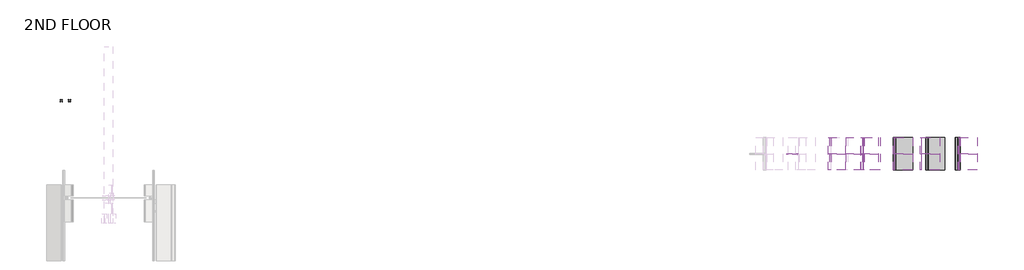
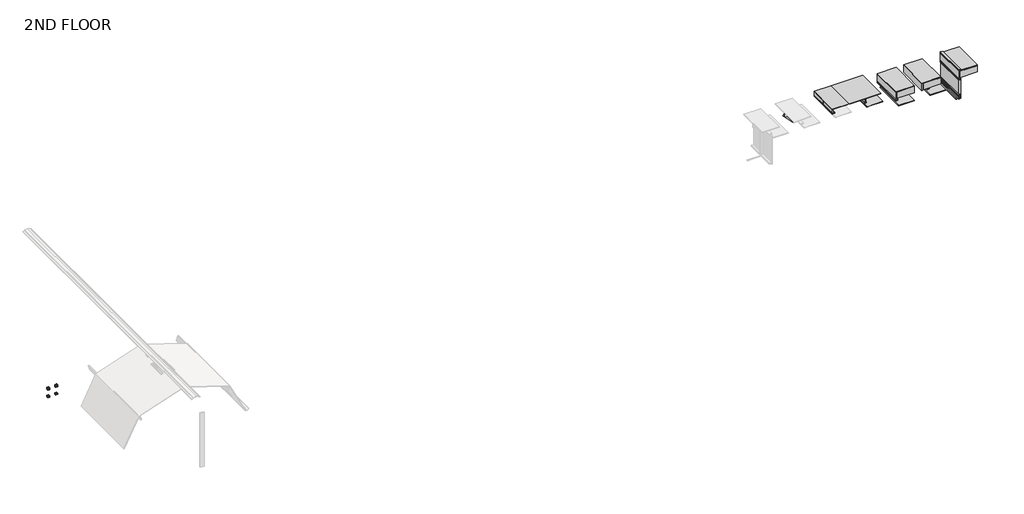
# One storey, part 2 of 2: 61 proxies.
"""IFC4 building model written with IfcOpenShell, lengths in millimetres."""

import ifcopenshell
import ifcopenshell.guid

model = None  # the IFC model being written
_history = None  # IfcOwnerHistory: only IFC2X3 demands one
_inside = {}  # id of a spatial element -> (the spatial element, [elements in it])
_under = {}  # id of a project, library or spatial element -> (it, [spatial elements below it])
_declared = {}  # id of a project -> (the project, [libraries it declares])
_typed = {}  # id of a type object -> (the type object, [elements of that type])
_made_of = {}  # id of a material, layer set ... -> (it, [elements and type objects made of it])


def new_model(schema):
    """Start an empty IFC model of exactly this schema.

    Asked for "IFC4X3", IfcOpenShell would pick the latest addendum, in which some entities
    have other attributes; the version numbers below select the first issue.
    IFC2X3 requires an IfcOwnerHistory on every rooted entity: one is made here for all.
    """
    global model, _history
    if schema == "IFC4X3":
        model = ifcopenshell.file(schema_version=(4, 3, 0, 0))
    else:
        model = ifcopenshell.file(schema=schema)
    _inside.clear()
    _under.clear()
    _declared.clear()
    _typed.clear()
    _made_of.clear()
    _history = None
    if model.schema == "IFC2X3":
        org = make("IfcOrganization", Name="unknown")
        user = make(
            "IfcPersonAndOrganization",
            ThePerson=make("IfcPerson", FamilyName="unknown"),
            TheOrganization=org,
        )
        app = make(
            "IfcApplication",
            ApplicationDeveloper=org,
            Version="unknown",
            ApplicationFullName="unknown",
            ApplicationIdentifier="unknown",
        )
        _history = make(
            "IfcOwnerHistory",
            OwningUser=user,
            OwningApplication=app,
            ChangeAction="ADDED",
            CreationDate=0,
        )
    return model


def make(cls, **values):
    """One entity of the class cls with the attributes given. An attribute that is None is left unset."""
    return model.create_entity(
        cls, **{name: value for name, value in values.items() if value is not None}
    )


def rooted(cls, **values):
    """An entity with a GlobalId (a new one), such as an element, a storey or a relation."""
    return make(cls, GlobalId=ifcopenshell.guid.new(), OwnerHistory=_history, **values)


def si_unit(unit_type, name, prefix=None):
    """IfcSIUnit, for example si_unit("LENGTHUNIT", "METRE", prefix="MILLI")."""
    return make("IfcSIUnit", UnitType=unit_type, Prefix=prefix, Name=name)


def assignment(units):
    """IfcUnitAssignment: the units of a project."""
    return None if units is None else make("IfcUnitAssignment", Units=units)


def point(xyz):
    """IfcCartesianPoint."""
    return None if xyz is None else make("IfcCartesianPoint", Coordinates=xyz)


def direction(xyz):
    """IfcDirection."""
    return None if xyz is None else make("IfcDirection", DirectionRatios=xyz)


def frame(location, z_axis=None, x_axis=None):
    """IfcAxis2Placement3D, a coordinate frame: its origin and axes. An axis left out is left unset."""
    return make(
        "IfcAxis2Placement3D",
        Location=point(location),
        Axis=direction(z_axis),
        RefDirection=direction(x_axis),
    )


def frame_2d(location, x_axis=None):
    """IfcAxis2Placement2D, a coordinate frame in the plane: its origin and x axis."""
    return make(
        "IfcAxis2Placement2D", Location=point(location), RefDirection=direction(x_axis)
    )


def origin():
    """The frame at (0, 0, 0) with its axes left unset."""
    return frame((0.0, 0.0, 0.0))


def origin_with_axes():
    """The frame at (0, 0, 0) with the z axis (0, 0, 1) and the x axis (1, 0, 0) written out."""
    return frame((0.0, 0.0, 0.0), z_axis=(0.0, 0.0, 1.0), x_axis=(1.0, 0.0, 0.0))


def origin_2d():
    """The frame at (0, 0) in the plane with its x axis left unset."""
    return frame_2d((0.0, 0.0))


def place(relative_to, where):
    """IfcLocalPlacement: puts the frame where relative to a parent placement (None: the world)."""
    return make(
        "IfcLocalPlacement", PlacementRelTo=relative_to, RelativePlacement=where
    )


def context(
    kind, dimensions, precision=None, world=None, true_north=None, identifier=None
):
    """IfcGeometricRepresentationContext, for example the 3D "Model" context."""
    return make(
        "IfcGeometricRepresentationContext",
        ContextIdentifier=identifier,
        ContextType=kind,
        CoordinateSpaceDimension=dimensions,
        Precision=precision,
        WorldCoordinateSystem=world,
        TrueNorth=true_north,
    )


def project(units=None, contexts=None):
    """IfcProject with its units and contexts."""
    return rooted(
        "IfcProject",
        Name="project",
        RepresentationContexts=contexts,
        UnitsInContext=assignment(units),
    )


def spatial(cls, under=None, at=None, **own):
    """A site, building, storey or space (cls), placed at a placement, below another one or the project."""
    s = rooted(cls, ObjectPlacement=at, **own)
    if under is not None:
        _under.setdefault(under.id(), (under, []))[1].append(s)
    return s


def polyline(points):
    """IfcPolyline through the points."""
    return make("IfcPolyline", Points=[point(p) for p in points])


def circle_curve(where, radius):
    """IfcCircle in the frame where."""
    return make("IfcCircle", Position=where, Radius=radius)


def trimmed(basis, trim1, trim2, sense, master):
    """IfcTrimmedCurve: the piece of a basis curve between two trims."""
    return make(
        "IfcTrimmedCurve",
        BasisCurve=basis,
        Trim1=trim1,
        Trim2=trim2,
        SenseAgreement=sense,
        MasterRepresentation=master,
    )


def segment(curve, same_sense, transition):
    """IfcCompositeCurveSegment."""
    return make(
        "IfcCompositeCurveSegment",
        Transition=transition,
        SameSense=same_sense,
        ParentCurve=curve,
    )


def composite_curve(segments, self_intersect=None):
    """IfcCompositeCurve: segments joined end to end."""
    return make("IfcCompositeCurve", Segments=segments, SelfIntersect=self_intersect)


def outline(outer, holes=None, kind="AREA"):
    """IfcArbitraryClosedProfileDef: a profile drawn as a closed curve; with holes, ...WithVoids."""
    if holes is None:
        return make("IfcArbitraryClosedProfileDef", ProfileType=kind, OuterCurve=outer)
    return make(
        "IfcArbitraryProfileDefWithVoids",
        ProfileType=kind,
        OuterCurve=outer,
        InnerCurves=holes,
    )


def extrude(swept, where, along, depth):
    """IfcExtrudedAreaSolid: the profile swept, set in the frame where, extruded along a direction by depth."""
    return make(
        "IfcExtrudedAreaSolid",
        SweptArea=swept,
        Position=where,
        ExtrudedDirection=direction(along),
        Depth=depth,
    )


def shape(context_of_items, identifier, shape_type, items):
    """IfcShapeRepresentation: the items that make up one representation, for example the "Body"."""
    return make(
        "IfcShapeRepresentation",
        ContextOfItems=context_of_items,
        RepresentationIdentifier=identifier,
        RepresentationType=shape_type,
        Items=items,
    )


def source(mapping_origin, context_of_items, identifier, shape_type, items):
    """IfcRepresentationMap: a shape defined once, which mapped items show again and again."""
    return make(
        "IfcRepresentationMap",
        MappingOrigin=mapping_origin,
        MappedRepresentation=shape(context_of_items, identifier, shape_type, items),
    )


def transform(
    local_origin,
    x_axis=None,
    y_axis=None,
    z_axis=None,
    scale=None,
    scale2=None,
    scale3=None,
    uniform=True,
):
    """IfcCartesianTransformationOperator3D, or its non-uniform kind. x_axis, y_axis, z_axis: its Axis1, 2, 3."""
    if uniform:
        return make(
            "IfcCartesianTransformationOperator3D",
            Axis1=direction(x_axis),
            Axis2=direction(y_axis),
            LocalOrigin=point(local_origin),
            Scale=scale,
            Axis3=direction(z_axis),
        )
    return make(
        "IfcCartesianTransformationOperator3DnonUniform",
        Axis1=direction(x_axis),
        Axis2=direction(y_axis),
        LocalOrigin=point(local_origin),
        Scale=scale,
        Axis3=direction(z_axis),
        Scale2=scale2,
        Scale3=scale3,
    )


def mapped(mapping_source, mapping_target):
    """IfcMappedItem: shows the shape of a source again, moved by a transform."""
    return make(
        "IfcMappedItem", MappingSource=mapping_source, MappingTarget=mapping_target
    )


def made_of(thing, what):
    """Note that an element or type object is made of a material, layer set ...; save() writes the relation."""
    if what is not None:
        _made_of.setdefault(what.id(), (what, []))[1].append(thing)
    return thing


def element(
    cls,
    number,
    at=None,
    inside=None,
    cuts=None,
    type_object=None,
    material=None,
    context=None,
    identifier="Body",
    shape_type=None,
    held_by="IfcProductDefinitionShape",
    body=None,
    shapes=None,
    **own,
):
    """One element of the class cls, such as IfcWall. Its Tag is "e" and its number.

    at: its placement. inside: the storey or other place that contains it. cuts: it is an
    opening in that element (IfcRelVoidsElement). A single representation is given by context,
    identifier, shape_type and body (its items); several are given by shapes. held_by: the class
    of the entity that holds the representations. save() writes the other relations.
    """
    e = rooted(cls, Tag="e%d" % number, ObjectPlacement=at, **own)
    if body is not None:
        shapes = [shape(context, identifier, shape_type, body)]
    if shapes is not None:
        e.Representation = make(held_by, Representations=shapes)
    if inside is not None:
        _inside.setdefault(inside.id(), (inside, []))[1].append(e)
    if cuts is not None:
        rooted(
            "IfcRelVoidsElement", RelatingBuildingElement=cuts, RelatedOpeningElement=e
        )
    if type_object is not None:
        _typed.setdefault(type_object.id(), (type_object, []))[1].append(e)
    return made_of(e, material)


def aggregate(whole, parts):
    """IfcRelAggregates: a whole, such as a stair, and the parts it consists of."""
    return rooted("IfcRelAggregates", RelatingObject=whole, RelatedObjects=parts)


def save(model, path):
    """Write the relations noted so far, then the file.

    IfcRelAggregates (storeys below a building ...), IfcRelContainedInSpatialStructure (elements
    in a storey), IfcRelDefinesByType, IfcRelAssociatesMaterial and IfcRelDeclares: one each for
    every whole, place, type object, material and project.
    """
    for whole, parts in _under.values():
        aggregate(whole, parts)
    for where, things in _inside.values():
        rooted(
            "IfcRelContainedInSpatialStructure",
            RelatedElements=things,
            RelatingStructure=where,
        )
    for kind, things in _typed.values():
        rooted("IfcRelDefinesByType", RelatedObjects=things, RelatingType=kind)
    for what, things in _made_of.values():
        rooted("IfcRelAssociatesMaterial", RelatedObjects=things, RelatingMaterial=what)
    for by, libraries in _declared.values():
        rooted("IfcRelDeclares", RelatingContext=by, RelatedDefinitions=libraries)
    model.write(path)


def generic_models_10_generic_models_1_ea081297(model_context):
    return source(origin(), model_context, "Body", "SweptSolid", [
        extrude(outline(polyline([(49758.6, 0.0), (49720.5, 0.0), (49720.5, 1219.2), (49758.6, 1219.2), (49758.6, 0.0)])), frame((0.0, 0.0, 5507.83125), z_axis=(0.0, 0.0, 1.0), x_axis=(1.0, 0.0, 0.0)), (0.0, 0.0, 1.0), 139.7),
    ])


def generic_models_102_generic_models_1_8a2dd616(model_context):
    return source(origin(), model_context, "Body", "SweptSolid", [
        extrude(outline(composite_curve([segment(polyline([(4498.578125, 52222.4), (4510.823229, 52207.8068534), (4508.6950617, 52206.021109), (4497.282664, 52219.621875), (4414.3677682, 52219.621875)]), True, "CONTINUOUS"), segment(trimmed(circle_curve(frame_2d((4414.4412941, 52217.6381931)), 1.9850441), [point((4414.3677682, 52219.621875))], [point((4412.45625, 52217.6381931))], True, "CARTESIAN"), True, "CONTINUOUS"), segment(polyline([(4412.45625, 52217.6381931), (4412.45625, 52023.9610661)]), True, "CONTINUOUS"), segment(trimmed(circle_curve(frame_2d((4414.4419899, 52023.9610661)), 1.9857399), [point((4412.45625, 52023.9610661))], [point((4414.3365981, 52021.978125))], True, "CARTESIAN"), True, "CONTINUOUS"), segment(polyline([(4414.3365981, 52021.978125), (4497.282664, 52021.978125), (4508.718285, 52035.6065673), (4510.8464522, 52033.820823), (4498.578125, 52019.2), (4414.440625, 52019.2)]), True, "CONTINUOUS"), segment(trimmed(circle_curve(frame_2d((4414.440625, 52023.9625)), 4.7625), [point((4414.440625, 52019.2))], [point((4409.678125, 52023.9625))], False, "CARTESIAN"), True, "CONTINUOUS"), segment(polyline([(4409.678125, 52023.9625), (4409.678125, 52217.6375)]), True, "CONTINUOUS"), segment(trimmed(circle_curve(frame_2d((4414.440625, 52217.6375)), 4.7625), [point((4409.678125, 52217.6375))], [point((4414.440625, 52222.4))], False, "CARTESIAN"), True, "CONTINUOUS"), segment(polyline([(4414.440625, 52222.4), (4498.578125, 52222.4)]), True, "CONTINUOUS")], self_intersect=False)), frame((0.0, 0.0, 0.0), z_axis=(0.0, 1.0, 0.0), x_axis=(0.0, 0.0, 1.0)), (0.0, 0.0, 1.0), 1219.2),
    ])


def generic_models_103_generic_models_1_250a6a11(model_context):
    return source(origin(), model_context, "Body", "SweptSolid", [
        extrude(outline(polyline([(49784.0, 0.0), (49695.1, 0.0), (49695.1, 1219.2), (49784.0, 1219.2), (49784.0, 0.0)])), frame((0.0, 0.0, 5264.15), z_axis=(0.0, 0.0, 1.0), x_axis=(1.0, 0.0, 0.0)), (0.0, 0.0, 1.0), 38.1),
    ])


def generic_models_104_generic_models_1_af33e5d9(model_context):
    return source(origin(), model_context, "Body", "SweptSolid", [
        extrude(outline(polyline([(52206.021109, 0.0), (52117.121109, 0.0), (52117.121109, 1219.2), (52206.021109, 1219.2), (52206.021109, 0.0)])), frame((0.0, 0.0, 4412.45625), z_axis=(0.0, 0.0, 1.0), x_axis=(1.0, 0.0, 0.0)), (0.0, 0.0, 1.0), 38.1),
    ])


def generic_models_108_generic_models_1_496acf5e(model_context):
    return source(origin(), model_context, "Body", "SweptSolid", [
        extrude(outline(polyline([(52216.05, 1219.2), (52216.05, 0.0), (52139.85, 0.0), (52139.85, 1219.2), (52216.05, 1219.2)])), frame((0.0, 0.0, 4570.4125), z_axis=(0.0, 0.0, 1.0), x_axis=(1.0, 0.0, 0.0)), (0.0, 0.0, 1.0), 565.15),
    ])


def generic_models_109_generic_models_1_8619d77b(model_context):
    return source(origin(), model_context, "Body", "SweptSolid", [
        extrude(outline(polyline([(51003.2, 0.0), (50914.3, 0.0), (50914.3, 1219.2), (51003.2, 1219.2), (51003.2, 0.0)])), frame((0.0, 0.0, 5184.378125), z_axis=(0.0, 0.0, 1.0), x_axis=(1.0, 0.0, 0.0)), (0.0, 0.0, 1.0), 38.1),
    ])


def generic_models_110_generic_models_1_6bdce9b6(model_context):
    return source(origin(), model_context, "Body", "SweptSolid", [
        extrude(outline(polyline([(51642.1451407, 1219.2), (51642.1451407, 0.0), (50914.3, 0.0), (50914.3, 1219.2), (51642.1451407, 1219.2)])), frame((0.0, 0.0, 5508.228125), z_axis=(0.0, 0.0, 1.0), x_axis=(1.0, 0.0, 0.0)), (0.0, 0.0, 1.0), 19.05),
    ])


def generic_models_112_generic_models_65_d168d7b0(model_context):
    return source(origin(), model_context, "Body", "SweptSolid", [
        extrude(outline(polyline([(50952.4, 592.1375), (50952.4, 630.2375), (51642.1451407, 630.2375), (51642.1451407, 592.1375), (50952.4, 592.1375)])), frame((0.0, 0.0, 5222.478125), z_axis=(0.0, 0.0, 1.0), x_axis=(1.0, 0.0, 0.0)), (0.0, 0.0, 1.0), 285.75),
    ])


def generic_models_113_generic_models_1_101608ab(model_context):
    return source(origin(), model_context, "Body", "SweptSolid", [
        extrude(outline(polyline([(52171.6, 0.0), (52133.5, 0.0), (52133.5, 1219.2), (52171.6, 1219.2), (52171.6, 0.0)])), frame((0.0, 0.0, 5222.478125), z_axis=(0.0, 0.0, 1.0), x_axis=(1.0, 0.0, 0.0)), (0.0, 0.0, 1.0), 285.75),
    ])


def generic_models_114_generic_models_1_a6fb1c2c(model_context):
    return source(origin(), model_context, "Body", "SweptSolid", [
        extrude(outline(polyline([(51642.1451407, 1219.2), (51642.1451407, 0.0), (50965.9242022, 0.0), (50965.9242022, 1219.2), (51642.1451407, 1219.2)])), frame((0.0, 0.0, 5237.6235034), z_axis=(0.0, 0.0, 1.0), x_axis=(1.0, 0.0, 0.0)), (0.0, 0.0, 1.0), 254.0),
    ])


def generic_models_12_generic_models_46_b8a9a4e8(model_context):
    return source(origin(), model_context, "Body", "SweptSolid", [
        extrude(outline(polyline([(49757.8505137, 0.0), (49721.1284797, 0.0), (49721.1284797, 1219.2), (49757.8505137, 1219.2), (49757.8505137, 0.0)])), frame((0.0, 0.0, 5505.7509163), z_axis=(0.0, 0.0, 1.0), x_axis=(1.0, 0.0, 0.0)), (0.0, 0.0, 1.0), 1.5875),
    ])


def generic_models_13_generic_models_65_9e643fb9(model_context):
    return source(origin(), model_context, "Body", "SweptSolid", [
        extrude(outline(polyline([(49128.3625, 592.1375), (49128.3625, 630.2375), (50347.5625, 630.2375), (50347.5625, 592.1375), (49128.3625, 592.1375)])), frame((0.0, 0.0, 5507.83125), z_axis=(0.0, 0.0, 1.0), x_axis=(1.0, 0.0, 0.0)), (0.0, 0.0, 1.0), 139.7),
    ])


def generic_models_14_generic_models_1_e8c90d4c(model_context):
    return source(origin(), model_context, "Body", "SweptSolid", [
        extrude(outline(polyline([(2277.1204978, 49799.875), (2239.0204978, 49799.875), (2239.0204978, 49825.275), (2240.6079978, 49825.275), (2240.6079978, 49801.4625), (2277.1204978, 49801.4625), (2277.1204978, 49799.875)])), frame((0.0, 0.0, 0.0), z_axis=(0.0, 1.0, 0.0), x_axis=(0.0, 0.0, 1.0)), (0.0, 0.0, 1.0), 1219.2),
    ])


def generic_models_22_generic_models_1_e5767157(model_context):
    return source(origin(), model_context, "Body", "SweptSolid", [
        extrude(outline(polyline([(2409.6091, 49800.66875), (2409.6091, 49799.875), (2407.0592364, 49799.875), (2405.4618473, 49749.075), (2404.6631527, 49749.075), (2403.0657636, 49799.875), (2400.5159, 49799.875), (2400.5159, 49800.66875), (2409.6091, 49800.66875)])), frame((0.0, 565.15, 0.0), z_axis=(0.0, 1.0, 0.0), x_axis=(0.0, 0.0, 1.0)), (0.0, 0.0, 1.0), 12.7),
    ])


def generic_models_233_generic_models_1_ae5bae41(model_context):
    return source(origin(), model_context, "Body", "SweptSolid", [
        extrude(outline(polyline([(48564.8, 0.0), (48475.9, 0.0), (48475.9, 1219.2), (48564.8, 1219.2), (48564.8, 0.0)])), frame((0.0, 0.0, 5467.35), z_axis=(0.0, 0.0, 1.0), x_axis=(1.0, 0.0, 0.0)), (0.0, 0.0, 1.0), 38.1),
    ])


def generic_models_236_generic_models_1_f8917e71(model_context):
    return source(origin(), model_context, "Body", "SweptSolid", [
        extrude(outline(polyline([(48507.65, 0.0), (48469.55, 0.0), (48469.55, 1219.2), (48507.65, 1219.2), (48507.65, 0.0)])), frame((0.0, 0.0, 5507.83125), z_axis=(0.0, 0.0, 1.0), x_axis=(1.0, 0.0, 0.0)), (0.0, 0.0, 1.0), 139.7),
    ])


def generic_models_237_generic_models_65_1df05f16(model_context):
    return source(origin(), model_context, "Body", "SweptSolid", [
        extrude(outline(polyline([(48469.55, 592.1375), (48469.55, 630.2375), (49128.3625, 630.2375), (49128.3625, 592.1375), (48469.55, 592.1375)])), frame((0.0, 0.0, 5507.83125), z_axis=(0.0, 0.0, 1.0), x_axis=(1.0, 0.0, 0.0)), (0.0, 0.0, 1.0), 139.7),
    ])


def generic_models_240_generic_models_1_611786cf(model_context):
    return source(origin(), model_context, "Body", "SweptSolid", [
        extrude(outline(polyline([(49128.3625, 1219.2), (49128.3625, 0.0), (48469.55, 0.0), (48469.55, 1219.2), (49128.3625, 1219.2)])), frame((0.0, 0.0, 5649.9125), z_axis=(0.0, 0.0, 1.0), x_axis=(1.0, 0.0, 0.0)), (0.0, 0.0, 1.0), 19.05),
    ])


def generic_models_267_generic_models_65_11354230(model_context):
    return source(origin(), model_context, "Body", "SweptSolid", [
        extrude(outline(polyline([(0.0, -38.1), (0.0, 0.0), (514.35, 0.0), (514.35, -38.1), (0.0, -38.1)])), frame((47276.4596037, 592.1375, 5202.484661), z_axis=(0.7071067811865633, 0.0, 0.7071067811865317), x_axis=(-0.7071067811865317, 0.0, 0.7071067811865633)), (0.0, 0.0, 1.0), 88.9),
    ])


def generic_models_29_generic_models_1_59087225(model_context):
    return source(origin(), model_context, "Body", "SweptSolid", [
        extrude(outline(polyline([(50347.5625, 1219.2), (50347.5625, 0.0), (49128.3625, 0.0), (49128.3625, 1219.2), (50347.5625, 1219.2)])), frame((0.0, 0.0, 5647.53125), z_axis=(0.0, 0.0, 1.0), x_axis=(1.0, 0.0, 0.0)), (0.0, 0.0, 1.0), 19.05),
    ])


def generic_models_226_generic_models_1_7dc37832(model_context):
    return source(origin(), model_context, "Body", "SweptSolid", [
        extrude(outline(polyline([(5263.35625, 49733.4159), (5263.35625, 49742.5091), (5264.15, 49742.5091), (5264.15, 49739.9592364), (5314.95, 49738.3618473), (5314.95, 49737.5631527), (5264.15, 49735.9657636), (5264.15, 49733.4159), (5263.35625, 49733.4159)])), frame((0.0, 565.15, 0.0), z_axis=(0.0, 1.0, 0.0), x_axis=(0.0, 0.0, 1.0)), (0.0, 0.0, 1.0), 12.7),
    ])


def generic_models_37_generic_models_1_916dd7c6(model_context):
    return source(origin(), model_context, "Body", "SweptSolid", [
        extrude(outline(polyline([(2409.6091, 49675.25625), (2400.5159, 49675.25625), (2400.5159, 49676.05), (2403.0657636, 49676.05), (2404.6631527, 49726.85), (2405.4618473, 49726.85), (2407.0592364, 49676.05), (2409.6091, 49676.05), (2409.6091, 49675.25625)])), frame((0.0, 565.15, 0.0), z_axis=(0.0, 1.0, 0.0), x_axis=(0.0, 0.0, 1.0)), (0.0, 0.0, 1.0), 12.7),
    ])


def generic_models_202_generic_models_1_0ad20a8b(model_context):
    return source(origin(), model_context, "Body", "SweptSolid", [
        extrude(outline(polyline([(2253.330428, 49813.3451407), (2242.217928, 49813.3451407), (2242.217928, 49826.0451407), (2234.280428, 49828.9341545), (2234.280428, 50422.9451407), (2253.330428, 50422.9451407), (2253.330428, 49813.3451407)])), frame((0.0, 0.0, 0.0), z_axis=(0.0, 1.0, 0.0), x_axis=(0.0, 0.0, 1.0)), (0.0, 0.0, 1.0), 1219.2),
    ])


def generic_models_71_generic_models_1_508a995f(model_context):
    return source(origin(), model_context, "Body", "SweptSolid", [
        extrude(outline(polyline([(50952.4, 0.0), (50914.3, 0.0), (50914.3, 1219.2), (50952.4, 1219.2), (50952.4, 0.0)])), frame((0.0, 0.0, 5222.478125), z_axis=(0.0, 0.0, 1.0), x_axis=(1.0, 0.0, 0.0)), (0.0, 0.0, 1.0), 285.75),
    ])


def generic_models_87_generic_models_1_55a64953(model_context):
    return source(origin(), model_context, "Body", "SweptSolid", [
        extrude(outline(polyline([(51968.4, 0.0), (51930.3, 0.0), (51930.3, 1219.2), (51968.4, 1219.2), (51968.4, 0.0)])), frame((0.0, 0.0, 5222.478125), z_axis=(0.0, 0.0, 1.0), x_axis=(1.0, 0.0, 0.0)), (0.0, 0.0, 1.0), 285.75),
    ])


def proxy_ced08073(model_context):
    return source(origin(), model_context, "Body", "SweptSolid", [
        extrude(outline(polyline([(-9.525, -5.4992613), (-9.525, 5.4992613), (0.0, 10.9985226), (9.525, 5.4992613), (9.525, -5.4992613), (0.0, -10.9985226), (-9.525, -5.4992613)])), frame((0.0, 0.0, -26.8882812), z_axis=(0.0, 0.0, 1.0), x_axis=(1.0, 0.0, 0.0)), (0.0, 0.0, 1.0), 12.7),
        extrude(outline(polyline([(-9.525, 5.4992613), (0.0, 10.9985226), (9.525, 5.4992613), (9.525, -5.4992613), (0.0, -10.9985226), (-9.525, -5.4992613), (-9.525, 5.4992613)])), origin_with_axes(), (0.0, 0.0, 1.0), 12.7),
        extrude(outline(composite_curve([segment(trimmed(circle_curve(origin_2d(), 6.35), [point((-6.35, 0.0))], [point((6.35, 0.0))], False, "CARTESIAN"), True, "CONTINUOUS"), segment(trimmed(circle_curve(origin_2d(), 6.35), [point((6.35, 0.0))], [point((-6.35, 0.0))], False, "CARTESIAN"), True, "CONTINUOUS")], self_intersect=False)), frame((0.0, 0.0, -38.1), z_axis=(0.0, 0.0, 1.0), x_axis=(1.0, 0.0, 0.0)), (0.0, 0.0, 1.0), 38.1),
    ])


def proxy_eacf5a22(model_context):
    return source(origin(), model_context, "Body", "SweptSolid", [
        extrude(outline(polyline([(-9.525, 5.4992613), (0.0, 10.9985226), (9.525, 5.4992613), (9.525, -5.4992613), (0.0, -10.9985226), (-9.525, -5.4992613), (-9.525, 5.4992613)])), frame((0.0, 0.0, -61.0195313), z_axis=(0.0, 0.0, 1.0), x_axis=(1.0, 0.0, 0.0)), (0.0, 0.0, 1.0), 8.73125),
        extrude(outline(polyline([(-9.525, -5.4992613), (-9.525, 5.4992613), (0.0, 10.9985226), (9.525, 5.4992613), (9.525, -5.4992613), (0.0, -10.9985226), (-9.525, -5.4992613)])), origin_with_axes(), (0.0, 0.0, 1.0), 8.73125),
        extrude(outline(composite_curve([segment(trimmed(circle_curve(origin_2d(), 6.35), [point((-6.35, 0.0))], [point((6.35, 0.0))], False, "CARTESIAN"), True, "CONTINUOUS"), segment(trimmed(circle_curve(origin_2d(), 6.35), [point((6.35, 0.0))], [point((-6.35, 0.0))], False, "CARTESIAN"), True, "CONTINUOUS")], self_intersect=False)), frame((0.0, 0.0, -63.5), z_axis=(0.0, 0.0, 1.0), x_axis=(1.0, 0.0, 0.0)), (0.0, 0.0, 1.0), 63.5),
    ])


model = new_model("IFC4")

# Units and contexts
model_context = context("Model", 3, world=origin())
ifc_project = project(units=[si_unit("LENGTHUNIT", "METRE", prefix="MILLI")], contexts=[model_context])

# Site, building, storey
site = spatial("IfcSite", under=ifc_project)
building = spatial("IfcBuilding", under=site)
storey = spatial("IfcBuildingStorey", under=building, Name="2ND FLOOR", Elevation=3984.625)

# Proxies
placement = place(None, origin())
generic_models_10_generic_models_1_shape = generic_models_10_generic_models_1_ea081297(model_context)
element("IfcBuildingElementProxy", 1, Name="Generic Models 10 : Generic Models 1", ObjectType="Generic Models 10 : Generic Models 1", at=placement, inside=storey, context=model_context, shape_type="MappedRepresentation", body=[
    mapped(generic_models_10_generic_models_1_shape, transform((0.0, 0.0, 0.0), x_axis=(1.0, 0.0, 0.0), y_axis=(0.0, 1.0, 0.0), z_axis=(0.0, 0.0, 1.0))),
])
generic_models_102_generic_models_1_shape = generic_models_102_generic_models_1_8a2dd616(model_context)
element("IfcBuildingElementProxy", 2, Name="Generic Models 102 : Generic Models 1", ObjectType="Generic Models 102 : Generic Models 1", at=placement, inside=storey, context=model_context, shape_type="MappedRepresentation", body=[
    mapped(generic_models_102_generic_models_1_shape, transform((1219.2, 0.0, 0.0), x_axis=(1.0, 0.0, 0.0), y_axis=(0.0, 1.0, 0.0), z_axis=(0.0, 0.0, 1.0))),
])
generic_models_103_generic_models_1_shape = generic_models_103_generic_models_1_250a6a11(model_context)
element("IfcBuildingElementProxy", 3, Name="Generic Models 103 : Generic Models 1", ObjectType="Generic Models 103 : Generic Models 1", at=placement, inside=storey, context=model_context, shape_type="MappedRepresentation", body=[
    mapped(generic_models_103_generic_models_1_shape, transform((3657.6, 0.0, -892.571875), x_axis=(1.0, 0.0, 0.0), y_axis=(0.0, 1.0, 0.0), z_axis=(0.0, 0.0, 1.0))),
])
generic_models_104_generic_models_1_shape = generic_models_104_generic_models_1_af33e5d9(model_context)
element("IfcBuildingElementProxy", 4, Name="Generic Models 104 : Generic Models 1", ObjectType="Generic Models 104 : Generic Models 1", at=placement, inside=storey, context=model_context, shape_type="MappedRepresentation", body=[
    mapped(generic_models_104_generic_models_1_shape, transform((1219.2, 0.0, 0.0), x_axis=(1.0, 0.0, 0.0), y_axis=(0.0, 1.0, 0.0), z_axis=(0.0, 0.0, 1.0))),
])
element("IfcBuildingElementProxy", 5, Name="Generic Models 105 : Generic Models 1", ObjectType="Generic Models 105 : Generic Models 1", at=placement, inside=storey, context=model_context, shape_type="MappedRepresentation", body=[
    mapped(generic_models_103_generic_models_1_shape, transform((3641.221109, 0.0, -813.59375), x_axis=(1.0, 0.0, 0.0), y_axis=(0.0, 1.0, 0.0), z_axis=(0.0, 0.0, 1.0))),
])
element("IfcBuildingElementProxy", 6, Name="Generic Models 106 : Generic Models 1", ObjectType="Generic Models 106 : Generic Models 1", at=placement, inside=storey, context=model_context, shape_type="MappedRepresentation", body=[
    mapped(generic_models_103_generic_models_1_shape, transform((3641.221109, 0.0, -775.49375), x_axis=(1.0, 0.0, 0.0), y_axis=(0.0, 1.0, 0.0), z_axis=(0.0, 0.0, 1.0))),
])
element("IfcBuildingElementProxy", 7, Name="Generic Models 107 : Generic Models 1", ObjectType="Generic Models 107 : Generic Models 1", at=placement, inside=storey, context=model_context, shape_type="MappedRepresentation", body=[
    mapped(generic_models_103_generic_models_1_shape, transform((3657.6, 0.0, -737.39375), x_axis=(1.0, 0.0, 0.0), y_axis=(0.0, 1.0, 0.0), z_axis=(0.0, 0.0, 1.0))),
])
generic_models_108_generic_models_1_shape = generic_models_108_generic_models_1_496acf5e(model_context)
element("IfcBuildingElementProxy", 8, Name="Generic Models 108 : Generic Models 1", ObjectType="Generic Models 108 : Generic Models 1", at=placement, inside=storey, context=model_context, shape_type="MappedRepresentation", body=[
    mapped(generic_models_108_generic_models_1_shape, transform((1219.2, 0.0, 0.0), x_axis=(1.0, 0.0, 0.0), y_axis=(0.0, 1.0, 0.0), z_axis=(0.0, 0.0, 1.0))),
])
generic_models_109_generic_models_1_shape = generic_models_109_generic_models_1_8619d77b(model_context)
element("IfcBuildingElementProxy", 9, Name="Generic Models 109 : Generic Models 1", ObjectType="Generic Models 109 : Generic Models 1", at=placement, inside=storey, context=model_context, shape_type="MappedRepresentation", body=[
    mapped(generic_models_109_generic_models_1_shape, transform((2438.4, 0.0, 0.0), x_axis=(1.0, 0.0, 0.0), y_axis=(0.0, 1.0, 0.0), z_axis=(0.0, 0.0, 1.0))),
])
generic_models_110_generic_models_1_shape = generic_models_110_generic_models_1_6bdce9b6(model_context)
element("IfcBuildingElementProxy", 10, Name="Generic Models 110 : Generic Models 1", ObjectType="Generic Models 110 : Generic Models 1", at=placement, inside=storey, context=model_context, shape_type="MappedRepresentation", body=[
    mapped(generic_models_110_generic_models_1_shape, transform((2438.4, 0.0, 0.0), x_axis=(1.0, 0.0, 0.0), y_axis=(0.0, 1.0, 0.0), z_axis=(0.0, 0.0, 1.0))),
])
element("IfcBuildingElementProxy", 11, Name="Generic Models 111 : Generic Models 1", ObjectType="Generic Models 111 : Generic Models 1", at=placement, inside=storey, context=model_context, shape_type="MappedRepresentation", body=[
    mapped(generic_models_109_generic_models_1_shape, transform((2438.4, 0.0, -38.1), x_axis=(1.0, 0.0, 0.0), y_axis=(0.0, 1.0, 0.0), z_axis=(0.0, 0.0, 1.0))),
])
generic_models_112_generic_models_65_shape = generic_models_112_generic_models_65_d168d7b0(model_context)
element("IfcBuildingElementProxy", 12, Name="Generic Models 112 : Generic Models 65", ObjectType="Generic Models 112 : Generic Models 65", at=placement, inside=storey, context=model_context, shape_type="MappedRepresentation", body=[
    mapped(generic_models_112_generic_models_65_shape, transform((2438.4, 0.0, 0.0), x_axis=(1.0, 0.0, 0.0), y_axis=(0.0, 1.0, 0.0), z_axis=(0.0, 0.0, 1.0))),
])
generic_models_113_generic_models_1_shape = generic_models_113_generic_models_1_101608ab(model_context)
element("IfcBuildingElementProxy", 13, Name="Generic Models 113 : Generic Models 1", ObjectType="Generic Models 113 : Generic Models 1", at=placement, inside=storey, context=model_context, shape_type="MappedRepresentation", body=[
    mapped(generic_models_113_generic_models_1_shape, transform((1219.2, 0.0, 0.0), x_axis=(1.0, 0.0, 0.0), y_axis=(0.0, 1.0, 0.0), z_axis=(0.0, 0.0, 1.0))),
])
generic_models_114_generic_models_1_shape = generic_models_114_generic_models_1_a6fb1c2c(model_context)
element("IfcBuildingElementProxy", 14, Name="Generic Models 114 : Generic Models 1", ObjectType="Generic Models 114 : Generic Models 1", at=placement, inside=storey, context=model_context, shape_type="MappedRepresentation", body=[
    mapped(generic_models_114_generic_models_1_shape, transform((2438.4, 0.0, 0.0), x_axis=(1.0, 0.0, 0.0), y_axis=(0.0, 1.0, 0.0), z_axis=(0.0, 0.0, 1.0))),
])
element("IfcBuildingElementProxy", 15, Name="Generic Models 115 : Generic Models 1", ObjectType="Generic Models 115 : Generic Models 1", at=placement, inside=storey, context=model_context, shape_type="MappedRepresentation", body=[
    mapped(generic_models_109_generic_models_1_shape, transform((2438.4, 0.0, 342.9), x_axis=(1.0, 0.0, 0.0), y_axis=(0.0, 1.0, 0.0), z_axis=(0.0, 0.0, 1.0))),
])
generic_models_12_generic_models_46_shape = generic_models_12_generic_models_46_b8a9a4e8(model_context)
element("IfcBuildingElementProxy", 16, Name="Generic Models 12 : Generic Models 46", ObjectType="Generic Models 12 : Generic Models 46", at=placement, inside=storey, context=model_context, shape_type="MappedRepresentation", body=[
    mapped(generic_models_12_generic_models_46_shape, transform((0.0, 0.0, 0.0), x_axis=(1.0, 0.0, 0.0), y_axis=(0.0, 1.0, 0.0), z_axis=(0.0, 0.0, 1.0))),
])
generic_models_13_generic_models_65_shape = generic_models_13_generic_models_65_9e643fb9(model_context)
element("IfcBuildingElementProxy", 17, Name="Generic Models 13 : Generic Models 65", ObjectType="Generic Models 13 : Generic Models 65", at=placement, inside=storey, context=model_context, shape_type="MappedRepresentation", body=[
    mapped(generic_models_13_generic_models_65_shape, transform((0.0, 0.0, 0.0), x_axis=(1.0, 0.0, 0.0), y_axis=(0.0, 1.0, 0.0), z_axis=(0.0, 0.0, 1.0))),
])
generic_models_14_generic_models_1_shape = generic_models_14_generic_models_1_e8c90d4c(model_context)
element("IfcBuildingElementProxy", 18, Name="Generic Models 14 : Generic Models 1", ObjectType="Generic Models 14 : Generic Models 1", at=placement, inside=storey, context=model_context, shape_type="MappedRepresentation", body=[
    mapped(generic_models_14_generic_models_1_shape, transform((0.0, 0.0, 3050.778125), x_axis=(1.0, 0.0, 0.0), y_axis=(0.0, 1.0, 0.0), z_axis=(0.0, 0.0, 1.0))),
])
generic_models_22_generic_models_1_shape = generic_models_22_generic_models_1_e5767157(model_context)
element("IfcBuildingElementProxy", 19, Name="Generic Models 22 : Generic Models 1", ObjectType="Generic Models 22 : Generic Models 1", at=placement, inside=storey, context=model_context, shape_type="MappedRepresentation", body=[
    mapped(generic_models_22_generic_models_1_shape, transform((0.0, 0.0, 3081.3375), x_axis=(1.0, 0.0, 0.0), y_axis=(0.0, 1.0, 0.0), z_axis=(0.0, 0.0, 1.0))),
])
generic_models_233_generic_models_1_shape = generic_models_233_generic_models_1_ae5bae41(model_context)
element("IfcBuildingElementProxy", 20, Name="Generic Models 233 : Generic Models 1", ObjectType="Generic Models 233 : Generic Models 1", at=placement, inside=storey, context=model_context, shape_type="MappedRepresentation", body=[
    mapped(generic_models_233_generic_models_1_shape, transform((0.0, 0.0, 0.0), x_axis=(1.0, 0.0, 0.0), y_axis=(0.0, 1.0, 0.0), z_axis=(0.0, 0.0, 1.0))),
])
generic_models_236_generic_models_1_shape = generic_models_236_generic_models_1_f8917e71(model_context)
element("IfcBuildingElementProxy", 21, Name="Generic Models 236 : Generic Models 1", ObjectType="Generic Models 236 : Generic Models 1", at=placement, inside=storey, context=model_context, shape_type="MappedRepresentation", body=[
    mapped(generic_models_236_generic_models_1_shape, transform((0.0, 0.0, 0.0), x_axis=(1.0, 0.0, 0.0), y_axis=(0.0, 1.0, 0.0), z_axis=(0.0, 0.0, 1.0))),
])
generic_models_237_generic_models_65_shape = generic_models_237_generic_models_65_1df05f16(model_context)
element("IfcBuildingElementProxy", 22, Name="Generic Models 237 : Generic Models 65", ObjectType="Generic Models 237 : Generic Models 65", at=placement, inside=storey, context=model_context, shape_type="MappedRepresentation", body=[
    mapped(generic_models_237_generic_models_65_shape, transform((0.0, 0.0, 0.0), x_axis=(1.0, 0.0, 0.0), y_axis=(0.0, 1.0, 0.0), z_axis=(0.0, 0.0, 1.0))),
])
generic_models_240_generic_models_1_shape = generic_models_240_generic_models_1_611786cf(model_context)
element("IfcBuildingElementProxy", 23, Name="Generic Models 240 : Generic Models 1", ObjectType="Generic Models 240 : Generic Models 1", at=placement, inside=storey, context=model_context, shape_type="MappedRepresentation", body=[
    mapped(generic_models_240_generic_models_1_shape, transform((0.0, 0.0, 0.0), x_axis=(1.0, 0.0, 0.0), y_axis=(0.0, 1.0, 0.0), z_axis=(0.0, 0.0, 1.0))),
])
element("IfcBuildingElementProxy", 24, Name="Generic Models 25 : Generic Models 46", ObjectType="Generic Models 25 : Generic Models 46", at=placement, inside=storey, context=model_context, shape_type="MappedRepresentation", body=[
    mapped(generic_models_12_generic_models_46_shape, transform((0.0, 0.0, 142.08125), x_axis=(1.0, 0.0, 0.0), y_axis=(0.0, 1.0, 0.0), z_axis=(0.0, 0.0, 1.0))),
])
generic_models_267_generic_models_65_shape = generic_models_267_generic_models_65_11354230(model_context)
element("IfcBuildingElementProxy", 25, Name="Generic Models 267 : Generic Models 65", ObjectType="Generic Models 267 : Generic Models 65", at=placement, inside=storey, context=model_context, shape_type="MappedRepresentation", body=[
    mapped(generic_models_267_generic_models_65_shape, transform((0.0, 0.0, 0.0), x_axis=(1.0, 0.0, 0.0), y_axis=(0.0, 1.0, 0.0), z_axis=(0.0, 0.0, 1.0))),
])
generic_models_29_generic_models_1_shape = generic_models_29_generic_models_1_59087225(model_context)
element("IfcBuildingElementProxy", 26, Name="Generic Models 29 : Generic Models 1", ObjectType="Generic Models 29 : Generic Models 1", at=placement, inside=storey, context=model_context, shape_type="MappedRepresentation", body=[
    mapped(generic_models_29_generic_models_1_shape, transform((0.0, 0.0, 2.38125), x_axis=(1.0, 0.0, 0.0), y_axis=(0.0, 1.0, 0.0), z_axis=(0.0, 0.0, 1.0))),
])
generic_models_226_generic_models_1_shape = generic_models_226_generic_models_1_7dc37832(model_context)
element("IfcBuildingElementProxy", 27, Name="Generic Models 39 : Generic Models 1", ObjectType="Generic Models 39 : Generic Models 1", at=placement, inside=storey, context=model_context, shape_type="MappedRepresentation", body=[
    mapped(generic_models_226_generic_models_1_shape, transform((0.0, 0.0, 203.2), x_axis=(1.0, 0.0, 0.0), y_axis=(0.0, 1.0, 0.0), z_axis=(0.0, 0.0, 1.0))),
])
generic_models_37_generic_models_1_shape = generic_models_37_generic_models_1_916dd7c6(model_context)
element("IfcBuildingElementProxy", 28, Name="Generic Models 47 : Generic Models 1", ObjectType="Generic Models 47 : Generic Models 1", at=placement, inside=storey, context=model_context, shape_type="MappedRepresentation", body=[
    mapped(generic_models_37_generic_models_1_shape, transform((3.175, 0.0, 3081.3375), x_axis=(1.0, 0.0, 0.0), y_axis=(0.0, 1.0, 0.0), z_axis=(0.0, 0.0, 1.0))),
])
generic_models_202_generic_models_1_shape = generic_models_202_generic_models_1_0ad20a8b(model_context)
element("IfcBuildingElementProxy", 29, Name="Generic Models 49 : Generic Models 1", ObjectType="Generic Models 49 : Generic Models 1", at=placement, inside=storey, context=model_context, shape_type="MappedRepresentation", body=[
    mapped(generic_models_202_generic_models_1_shape, transform((0.0, 0.0, 3050.778125), x_axis=(1.0, 0.0, 0.0), y_axis=(0.0, 1.0, 0.0), z_axis=(0.0, 0.0, 1.0))),
])
element("IfcBuildingElementProxy", 30, Name="Generic Models 54 : Generic Models 1", ObjectType="Generic Models 54 : Generic Models 1", at=placement, inside=storey, context=model_context, shape_type="MappedRepresentation", body=[
    mapped(generic_models_14_generic_models_1_shape, transform((1219.2, 0.0, 2676.128125), x_axis=(1.0, 0.0, 0.0), y_axis=(0.0, 1.0, 0.0), z_axis=(0.0, 0.0, 1.0))),
])
element("IfcBuildingElementProxy", 31, Name="Generic Models 59 : Generic Models 65", ObjectType="Generic Models 59 : Generic Models 65", at=placement, inside=storey, context=model_context, shape_type="MappedRepresentation", body=[
    mapped(generic_models_112_generic_models_65_shape, transform((0.0, 0.0, 0.0), x_axis=(1.0, 0.0, 0.0), y_axis=(0.0, 1.0, 0.0), z_axis=(0.0, 0.0, 1.0))),
])
element("IfcBuildingElementProxy", 32, Name="Generic Models 6 : Generic Models 1", ObjectType="Generic Models 6 : Generic Models 1", at=placement, inside=storey, context=model_context, shape_type="MappedRepresentation", body=[
    mapped(generic_models_103_generic_models_1_shape, transform((0.0, 0.0, 203.2), x_axis=(1.0, 0.0, 0.0), y_axis=(0.0, 1.0, 0.0), z_axis=(0.0, 0.0, 1.0))),
])
element("IfcBuildingElementProxy", 33, Name="Generic Models 62 : Generic Models 1", ObjectType="Generic Models 62 : Generic Models 1", at=placement, inside=storey, context=model_context, shape_type="MappedRepresentation", body=[
    mapped(generic_models_202_generic_models_1_shape, transform((1219.2, 0.0, 2676.128125), x_axis=(1.0, 0.0, 0.0), y_axis=(0.0, 1.0, 0.0), z_axis=(0.0, 0.0, 1.0))),
])
element("IfcBuildingElementProxy", 34, Name="Generic Models 64 : Generic Models 1", ObjectType="Generic Models 64 : Generic Models 1", at=placement, inside=storey, context=model_context, shape_type="MappedRepresentation", body=[
    mapped(generic_models_109_generic_models_1_shape, transform((0.0, 0.0, 0.0), x_axis=(1.0, 0.0, 0.0), y_axis=(0.0, 1.0, 0.0), z_axis=(0.0, 0.0, 1.0))),
])
element("IfcBuildingElementProxy", 35, Name="Generic Models 66 : Generic Models 1", ObjectType="Generic Models 66 : Generic Models 1", at=placement, inside=storey, context=model_context, shape_type="MappedRepresentation", body=[
    mapped(generic_models_110_generic_models_1_shape, transform((0.0, 0.0, 0.0), x_axis=(1.0, 0.0, 0.0), y_axis=(0.0, 1.0, 0.0), z_axis=(0.0, 0.0, 1.0))),
])
element("IfcBuildingElementProxy", 36, Name="Generic Models 70 : Generic Models 1", ObjectType="Generic Models 70 : Generic Models 1", at=placement, inside=storey, context=model_context, shape_type="MappedRepresentation", body=[
    mapped(generic_models_109_generic_models_1_shape, transform((0.0, 0.0, -38.1), x_axis=(1.0, 0.0, 0.0), y_axis=(0.0, 1.0, 0.0), z_axis=(0.0, 0.0, 1.0))),
])
generic_models_71_generic_models_1_shape = generic_models_71_generic_models_1_508a995f(model_context)
element("IfcBuildingElementProxy", 37, Name="Generic Models 71 : Generic Models 1", ObjectType="Generic Models 71 : Generic Models 1", at=placement, inside=storey, context=model_context, shape_type="MappedRepresentation", body=[
    mapped(generic_models_71_generic_models_1_shape, transform((0.0, 0.0, 0.0), x_axis=(1.0, 0.0, 0.0), y_axis=(0.0, 1.0, 0.0), z_axis=(0.0, 0.0, 1.0))),
])
element("IfcBuildingElementProxy", 38, Name="Generic Models 72 : Generic Models 1", ObjectType="Generic Models 72 : Generic Models 1", at=placement, inside=storey, context=model_context, shape_type="MappedRepresentation", body=[
    mapped(generic_models_114_generic_models_1_shape, transform((0.0, 0.0, 0.0), x_axis=(1.0, 0.0, 0.0), y_axis=(0.0, 1.0, 0.0), z_axis=(0.0, 0.0, 1.0))),
])
element("IfcBuildingElementProxy", 39, Name="Generic Models 75 : Generic Models 1", ObjectType="Generic Models 75 : Generic Models 1", at=placement, inside=storey, context=model_context, shape_type="MappedRepresentation", body=[
    mapped(generic_models_14_generic_models_1_shape, transform((2438.4, 0.0, 2676.128125), x_axis=(1.0, 0.0, 0.0), y_axis=(0.0, 1.0, 0.0), z_axis=(0.0, 0.0, 1.0))),
])
element("IfcBuildingElementProxy", 40, Name="Generic Models 79 : Generic Models 1", ObjectType="Generic Models 79 : Generic Models 1", at=placement, inside=storey, context=model_context, shape_type="MappedRepresentation", body=[
    mapped(generic_models_202_generic_models_1_shape, transform((2438.4, 0.0, 2676.128125), x_axis=(1.0, 0.0, 0.0), y_axis=(0.0, 1.0, 0.0), z_axis=(0.0, 0.0, 1.0))),
])
element("IfcBuildingElementProxy", 41, Name="Generic Models 81 : Generic Models 1", ObjectType="Generic Models 81 : Generic Models 1", at=placement, inside=storey, context=model_context, shape_type="MappedRepresentation", body=[
    mapped(generic_models_109_generic_models_1_shape, transform((1219.2, 0.0, 0.0), x_axis=(1.0, 0.0, 0.0), y_axis=(0.0, 1.0, 0.0), z_axis=(0.0, 0.0, 1.0))),
])
element("IfcBuildingElementProxy", 42, Name="Generic Models 82 : Generic Models 1", ObjectType="Generic Models 82 : Generic Models 1", at=placement, inside=storey, context=model_context, shape_type="MappedRepresentation", body=[
    mapped(generic_models_110_generic_models_1_shape, transform((1016.0, 0.0, 0.0), x_axis=(1.0, 0.0, 0.0), y_axis=(0.0, 1.0, 0.0), z_axis=(0.0, 0.0, 1.0))),
])
element("IfcBuildingElementProxy", 43, Name="Generic Models 86 : Generic Models 65", ObjectType="Generic Models 86 : Generic Models 65", at=placement, inside=storey, context=model_context, shape_type="MappedRepresentation", body=[
    mapped(generic_models_112_generic_models_65_shape, transform((1016.0, 0.0, 0.0), x_axis=(1.0, 0.0, 0.0), y_axis=(0.0, 1.0, 0.0), z_axis=(0.0, 0.0, 1.0))),
])
generic_models_87_generic_models_1_shape = generic_models_87_generic_models_1_55a64953(model_context)
element("IfcBuildingElementProxy", 44, Name="Generic Models 87 : Generic Models 1", ObjectType="Generic Models 87 : Generic Models 1", at=placement, inside=storey, context=model_context, shape_type="MappedRepresentation", body=[
    mapped(generic_models_87_generic_models_1_shape, transform((0.0, 0.0, 0.0), x_axis=(1.0, 0.0, 0.0), y_axis=(0.0, 1.0, 0.0), z_axis=(0.0, 0.0, 1.0))),
])
element("IfcBuildingElementProxy", 45, Name="Generic Models 88 : Generic Models 1", ObjectType="Generic Models 88 : Generic Models 1", at=placement, inside=storey, context=model_context, shape_type="MappedRepresentation", body=[
    mapped(generic_models_114_generic_models_1_shape, transform((1016.0, 0.0, 0.0), x_axis=(1.0, 0.0, 0.0), y_axis=(0.0, 1.0, 0.0), z_axis=(0.0, 0.0, 1.0))),
])
proxy_shape = proxy_ced08073(model_context)
element("IfcBuildingElementProxy", 46, Name="Lag Bolt : 1/2\" X 1 1/2\"", ObjectType="Lag Bolt : 1/2\" X 1 1/2\"", at=placement, inside=storey, context=model_context, shape_type="MappedRepresentation", body=[
    mapped(proxy_shape, transform((19698.4870052, 2642.8615366, 2431.4546875), x_axis=(1.0, 0.0, 0.0), y_axis=(0.0, -1.0, 0.0), z_axis=(0.0, 0.0, -1.0))),
])
element("IfcBuildingElementProxy", 47, Name="Lag Bolt : 1/2\" X 1 1/2\"", ObjectType="Lag Bolt : 1/2\" X 1 1/2\"", at=placement, inside=storey, context=model_context, shape_type="MappedRepresentation", body=[
    mapped(proxy_shape, transform((19634.9870052, 2642.8615366, 2431.4546875), x_axis=(1.0, 0.0, 0.0), y_axis=(0.0, -1.0, 0.0), z_axis=(0.0, 0.0, -1.0))),
])
element("IfcBuildingElementProxy", 48, Name="Lag Bolt : 1/2\" X 1 1/2\"", ObjectType="Lag Bolt : 1/2\" X 1 1/2\"", at=placement, inside=storey, context=model_context, shape_type="MappedRepresentation", body=[
    mapped(proxy_shape, transform((19698.4870052, 2579.3615366, 2431.4546875), x_axis=(1.0, 0.0, 0.0), y_axis=(0.0, -1.0, 0.0), z_axis=(0.0, 0.0, -1.0))),
])
element("IfcBuildingElementProxy", 49, Name="Lag Bolt : 1/2\" X 1 1/2\"", ObjectType="Lag Bolt : 1/2\" X 1 1/2\"", at=placement, inside=storey, context=model_context, shape_type="MappedRepresentation", body=[
    mapped(proxy_shape, transform((19634.9870052, 2579.3615366, 2431.4546875), x_axis=(1.0, 0.0, 0.0), y_axis=(0.0, -1.0, 0.0), z_axis=(0.0, 0.0, -1.0))),
])
element("IfcBuildingElementProxy", 50, Name="Lag Bolt : 1/2\" X 1 1/2\"", ObjectType="Lag Bolt : 1/2\" X 1 1/2\"", at=placement, inside=storey, context=model_context, shape_type="MappedRepresentation", body=[
    mapped(proxy_shape, transform((20003.2870052, 2642.8615366, 2431.4546875), x_axis=(1.0, 0.0, 0.0), y_axis=(0.0, -1.0, 0.0), z_axis=(0.0, 0.0, -1.0))),
])
element("IfcBuildingElementProxy", 51, Name="Lag Bolt : 1/2\" X 1 1/2\"", ObjectType="Lag Bolt : 1/2\" X 1 1/2\"", at=placement, inside=storey, context=model_context, shape_type="MappedRepresentation", body=[
    mapped(proxy_shape, transform((19939.7870052, 2642.8615366, 2431.4546875), x_axis=(1.0, 0.0, 0.0), y_axis=(0.0, -1.0, 0.0), z_axis=(0.0, 0.0, -1.0))),
])
element("IfcBuildingElementProxy", 52, Name="Lag Bolt : 1/2\" X 1 1/2\"", ObjectType="Lag Bolt : 1/2\" X 1 1/2\"", at=placement, inside=storey, context=model_context, shape_type="MappedRepresentation", body=[
    mapped(proxy_shape, transform((20003.2870052, 2579.3615366, 2431.4546875), x_axis=(1.0, 0.0, 0.0), y_axis=(0.0, -1.0, 0.0), z_axis=(0.0, 0.0, -1.0))),
])
element("IfcBuildingElementProxy", 53, Name="Lag Bolt : 1/2\" X 1 1/2\"", ObjectType="Lag Bolt : 1/2\" X 1 1/2\"", at=placement, inside=storey, context=model_context, shape_type="MappedRepresentation", body=[
    mapped(proxy_shape, transform((19939.7870052, 2579.3615366, 2431.4546875), x_axis=(1.0, 0.0, 0.0), y_axis=(0.0, -1.0, 0.0), z_axis=(0.0, 0.0, -1.0))),
])
proxy_2_shape = proxy_eacf5a22(model_context)
element("IfcBuildingElementProxy", 54, Name="Lag Bolt : 1/2\" x 2 1/2\"", ObjectType="Lag Bolt : 1/2\" x 2 1/2\"", at=placement, inside=storey, context=model_context, shape_type="MappedRepresentation", body=[
    mapped(proxy_2_shape, transform((19698.4870052, 2642.8615366, 2789.0390625), x_axis=(1.0, 0.0, 0.0), y_axis=(0.0, 1.0, 0.0), z_axis=(0.0, 0.0, 1.0))),
])
element("IfcBuildingElementProxy", 55, Name="Lag Bolt : 1/2\" x 2 1/2\"", ObjectType="Lag Bolt : 1/2\" x 2 1/2\"", at=placement, inside=storey, context=model_context, shape_type="MappedRepresentation", body=[
    mapped(proxy_2_shape, transform((19634.9870052, 2642.8615366, 2789.0390625), x_axis=(1.0, 0.0, 0.0), y_axis=(0.0, 1.0, 0.0), z_axis=(0.0, 0.0, 1.0))),
])
element("IfcBuildingElementProxy", 56, Name="Lag Bolt : 1/2\" x 2 1/2\"", ObjectType="Lag Bolt : 1/2\" x 2 1/2\"", at=placement, inside=storey, context=model_context, shape_type="MappedRepresentation", body=[
    mapped(proxy_2_shape, transform((19698.4870052, 2579.3615366, 2789.0390625), x_axis=(1.0, 0.0, 0.0), y_axis=(0.0, 1.0, 0.0), z_axis=(0.0, 0.0, 1.0))),
])
element("IfcBuildingElementProxy", 57, Name="Lag Bolt : 1/2\" x 2 1/2\"", ObjectType="Lag Bolt : 1/2\" x 2 1/2\"", at=placement, inside=storey, context=model_context, shape_type="MappedRepresentation", body=[
    mapped(proxy_2_shape, transform((19634.9870052, 2579.3615366, 2789.0390625), x_axis=(1.0, 0.0, 0.0), y_axis=(0.0, 1.0, 0.0), z_axis=(0.0, 0.0, 1.0))),
])
element("IfcBuildingElementProxy", 58, Name="Lag Bolt : 1/2\" x 2 1/2\"", ObjectType="Lag Bolt : 1/2\" x 2 1/2\"", at=placement, inside=storey, context=model_context, shape_type="MappedRepresentation", body=[
    mapped(proxy_2_shape, transform((20003.2870052, 2642.8615366, 2789.0390625), x_axis=(1.0, 0.0, 0.0), y_axis=(0.0, 1.0, 0.0), z_axis=(0.0, 0.0, 1.0))),
])
element("IfcBuildingElementProxy", 59, Name="Lag Bolt : 1/2\" x 2 1/2\"", ObjectType="Lag Bolt : 1/2\" x 2 1/2\"", at=placement, inside=storey, context=model_context, shape_type="MappedRepresentation", body=[
    mapped(proxy_2_shape, transform((19939.7870052, 2642.8615366, 2789.0390625), x_axis=(1.0, 0.0, 0.0), y_axis=(0.0, 1.0, 0.0), z_axis=(0.0, 0.0, 1.0))),
])
element("IfcBuildingElementProxy", 60, Name="Lag Bolt : 1/2\" x 2 1/2\"", ObjectType="Lag Bolt : 1/2\" x 2 1/2\"", at=placement, inside=storey, context=model_context, shape_type="MappedRepresentation", body=[
    mapped(proxy_2_shape, transform((20003.2870052, 2579.3615366, 2789.0390625), x_axis=(1.0, 0.0, 0.0), y_axis=(0.0, 1.0, 0.0), z_axis=(0.0, 0.0, 1.0))),
])
element("IfcBuildingElementProxy", 61, Name="Lag Bolt : 1/2\" x 2 1/2\"", ObjectType="Lag Bolt : 1/2\" x 2 1/2\"", at=placement, inside=storey, context=model_context, shape_type="MappedRepresentation", body=[
    mapped(proxy_2_shape, transform((19939.7870052, 2579.3615366, 2789.0390625), x_axis=(1.0, 0.0, 0.0), y_axis=(0.0, 1.0, 0.0), z_axis=(0.0, 0.0, 1.0))),
])

save(model, "model.ifc")

# Revit data of these elements
# Project information
#   Project Issue Date = "06/12/2018"
#   Project Status = "Project Status"
#   Client Name = "Owner"
#   Project Address = "39900 60TH ST BURLINGTON 53105"
#   Project Name = "RIVER VALLEY RANCH"
#   Project Number = "Project Number"
# Grids (mm)
#   "XX": line (4648.2, 7403.273) -> (4648.2, -3214.464)
#   "YY": line (-1465.333, 2057.4) -> (11893.622, 2057.4)
# Type "Lag Bolt : 1/2\" X 1 1/2\""
#   Thickness_of_Substrate [instance default] = 0' - 1"
#   Side = 0' - 0 111/256"
#   Radius = 0' - 0 1/4"
#   Length = 0' - 1 1/2"
#   Head Size = 0' - 0 3/4"
#   Head Radius = 0' - 0 3/8"
#   Head Height = 0' - 0 1/2"
#   Diameter = 0' - 0 1/2"
#   Default Elevation = 4' - 0"
#   Nut_Visibility [instance default] = yes
#   Bolt Material (Size) [instance default] = 1/2" X 5" LAG BOLT (THRU BOLT IF PLATE ON OPP. SIDE OF STRUCT MEMBER)
# Type "Lag Bolt : 1/2\" x 2 1/2\""
#   Thickness_of_Substrate [instance default] = 0' - 1"
#   Side = 0' - 0 111/256"
#   Radius = 0' - 0 1/4"
#   Length = 0' - 2 1/2"
#   Head Size = 0' - 0 3/4"
#   Head Radius = 0' - 0 3/8"
#   Head Height = 0' - 0 11/32"
#   Diameter = 0' - 0 1/2"
#   Default Elevation = 4' - 0"
#   Nut_Visibility [instance default] = yes
#   Bolt Material (Size) [instance default] = STRUCTURAL BOLTS (PAINT TO MATCH STEEL FINISH)
# Element 1 (IfcBuildingElementProxy, "Generic Models 10 : Generic Models 1")
#   Phase Created = _ZAVE_2
#   Materials on its faces: "2X BLOCKING - LOCATED AT GRAB BARS, WALL HUNG CABINETS, ETC.)"
# Element 2 (IfcBuildingElementProxy, "Generic Models 102 : Generic Models 1")
#   Phase Created = _ZAVE_2
#   Materials on its faces: "EXISTING GIRT"
# Element 3 (IfcBuildingElementProxy, "Generic Models 103 : Generic Models 1")
#   Phase Created = _ZAVE_2
#   Materials on its faces: "2X WOOD HEADER ATTACHED TO EXISTING JOIST"
# Element 4 (IfcBuildingElementProxy, "Generic Models 104 : Generic Models 1")
#   Phase Created = _ZAVE_2
#   Materials on its faces: "WOOD BLOCKING - SIZE AS NECESSARY"
# Element 5 (IfcBuildingElementProxy, "Generic Models 105 : Generic Models 1")
#   Phase Created = _ZAVE_2
#   Materials on its faces: "2X WOOD HEADER ATTACHED TO EXISTING JOIST"
# Element 6 (IfcBuildingElementProxy, "Generic Models 106 : Generic Models 1")
#   Phase Created = _ZAVE_2
#   Materials on its faces: "2X WOOD HEADER ATTACHED TO EXISTING JOIST"
# Element 7 (IfcBuildingElementProxy, "Generic Models 107 : Generic Models 1")
#   Phase Created = _ZAVE_2
#   Materials on its faces: "2X WOOD HEADER ATTACHED TO EXISTING JOIST"
# Element 8 (IfcBuildingElementProxy, "Generic Models 108 : Generic Models 1")
#   Phase Created = _ZAVE_2
#   Materials on its faces: "(S) SOUND BATT. INSULATION (THICKNESS TO MATCH WALL DEPTH)"
# Element 9 (IfcBuildingElementProxy, "Generic Models 109 : Generic Models 1")
#   Phase Created = _ZAVE_2
#   Materials on its faces: "DOUBLE 2X WOOD TOP PLATE"
# Element 10 (IfcBuildingElementProxy, "Generic Models 110 : Generic Models 1")
#   Phase Created = _ZAVE_2
#   Materials on its faces: "3/4\" CDX PLYWOOD"
# Element 11 (IfcBuildingElementProxy, "Generic Models 111 : Generic Models 1")
#   Phase Created = _ZAVE_2
#   Materials on its faces: "DOUBLE 2X WOOD TOP PLATE"
# Element 12 (IfcBuildingElementProxy, "Generic Models 112 : Generic Models 65")
#   Phase Created = _ZAVE_2
#   Materials on its faces: "WOOD JOIST AS SPECIFIED"
# Element 13 (IfcBuildingElementProxy, "Generic Models 113 : Generic Models 1")
#   Phase Created = _ZAVE_2
#   Materials on its faces: "RIM BOARD - SIZE TO MATCH JOIST DEPTH"
# Element 14 (IfcBuildingElementProxy, "Generic Models 114 : Generic Models 1")
#   Phase Created = _ZAVE_2
#   Materials on its faces: "SOUND BATT. INSULATION"
# Element 15 (IfcBuildingElementProxy, "Generic Models 115 : Generic Models 1")
#   Phase Created = _ZAVE_2
#   Materials on its faces: "DOUBLE 2X WOOD TOP PLATE"
# Element 16 (IfcBuildingElementProxy, "Generic Models 12 : Generic Models 46")
#   Phase Created = _ZAVE_2
#   Materials on its faces: "SET IN BED OF SEALANT"
# Element 17 (IfcBuildingElementProxy, "Generic Models 13 : Generic Models 65")
#   Phase Created = _ZAVE_2
#   Materials on its faces: "WOOD JOIST AS SPECIFIED"
# Element 18 (IfcBuildingElementProxy, "Generic Models 14 : Generic Models 1")
#   Phase Created = _ZAVE_2
#   Materials on its faces: "CEILING TRACK AS SCHEDULED"
# Element 19 (IfcBuildingElementProxy, "Generic Models 22 : Generic Models 1")
#   Phase Created = _ZAVE_2
#   Materials on its faces: "ATTACH GYPSUM BOARD TO STUDS AND NOT TO TOP TRACK"
# Element 20 (IfcBuildingElementProxy, "Generic Models 233 : Generic Models 1")
#   Phase Created = _ZAVE_2
#   Materials on its faces: "2X WOOD HEADER ATTACHED TO EXISTING JOIST"
# Element 21 (IfcBuildingElementProxy, "Generic Models 236 : Generic Models 1")
#   Phase Created = _ZAVE_2
#   Materials on its faces: "EXISTING RIM BOARD OR JOIST"
# Element 22 (IfcBuildingElementProxy, "Generic Models 237 : Generic Models 65")
#   Phase Created = _ZAVE_2
#   Materials on its faces: "WOOD JOIST AS SPECIFIED"
# Element 23 (IfcBuildingElementProxy, "Generic Models 240 : Generic Models 1")
#   Phase Created = _ZAVE_2
#   Materials on its faces: "EXISTING SUBSTRATE"
# Element 24 (IfcBuildingElementProxy, "Generic Models 25 : Generic Models 46")
#   Phase Created = _ZAVE_2
#   Materials on its faces: "SET IN BED OF SEALANT"
# Element 25 (IfcBuildingElementProxy, "Generic Models 267 : Generic Models 65")
#   Phase Created = _ZAVE_2
#   Materials on its faces: "DIAGONAL BRACING AS REQUIRED"
# Element 26 (IfcBuildingElementProxy, "Generic Models 29 : Generic Models 1")
#   Phase Created = _ZAVE_2
#   Materials on its faces: "SUBSTRATE AS SCHEDULED"
# Element 27 (IfcBuildingElementProxy, "Generic Models 39 : Generic Models 1")
#   Phase Created = _ZAVE_2
#   Materials on its faces: "METAL RUNNER CHANNEL; FASTEN @ 24\" O.C."
# Element 28 (IfcBuildingElementProxy, "Generic Models 47 : Generic Models 1")
#   Phase Created = _ZAVE_2
#   Materials on its faces: "ATTACH GYPSUM BOARD TO STUDS AND NOT TO TOP TRACK"
# Element 29 (IfcBuildingElementProxy, "Generic Models 49 : Generic Models 1")
#   Phase Created = _ZAVE_2
#   Materials on its faces: "CEILING AS SCHEDULED"
# Element 30 (IfcBuildingElementProxy, "Generic Models 54 : Generic Models 1")
#   Phase Created = _ZAVE_2
#   Materials on its faces: "CEILING TRACK AS SCHEDULED"
# Element 31 (IfcBuildingElementProxy, "Generic Models 59 : Generic Models 65")
#   Phase Created = _ZAVE_2
#   Materials on its faces: "WOOD JOIST AS SPECIFIED"
# Element 32 (IfcBuildingElementProxy, "Generic Models 6 : Generic Models 1")
#   Phase Created = _ZAVE_2
#   Materials on its faces: "2X WOOD HEADER ATTACHED TO EXISTING JOIST"
# Element 33 (IfcBuildingElementProxy, "Generic Models 62 : Generic Models 1")
#   Phase Created = _ZAVE_2
#   Materials on its faces: "CEILING AS SCHEDULED"
# Element 34 (IfcBuildingElementProxy, "Generic Models 64 : Generic Models 1")
#   Phase Created = _ZAVE_2
#   Materials on its faces: "DOUBLE 2X WOOD TOP PLATE"
# Element 35 (IfcBuildingElementProxy, "Generic Models 66 : Generic Models 1")
#   Phase Created = _ZAVE_2
#   Materials on its faces: "3/4\" CDX PLYWOOD"
# Element 36 (IfcBuildingElementProxy, "Generic Models 70 : Generic Models 1")
#   Phase Created = _ZAVE_2
#   Materials on its faces: "DOUBLE 2X WOOD TOP PLATE"
# Element 37 (IfcBuildingElementProxy, "Generic Models 71 : Generic Models 1")
#   Phase Created = _ZAVE_2
#   Materials on its faces: "DOUBLE 2X WOOD TOP PLATE"
# Element 38 (IfcBuildingElementProxy, "Generic Models 72 : Generic Models 1")
#   Phase Created = _ZAVE_2
#   Materials on its faces: "SOUND BATT. INSULATION"
# Element 39 (IfcBuildingElementProxy, "Generic Models 75 : Generic Models 1")
#   Phase Created = _ZAVE_2
#   Materials on its faces: "CEILING TRACK AS SCHEDULED"
# Element 40 (IfcBuildingElementProxy, "Generic Models 79 : Generic Models 1")
#   Phase Created = _ZAVE_2
#   Materials on its faces: "CEILING AS SCHEDULED"
# Element 41 (IfcBuildingElementProxy, "Generic Models 81 : Generic Models 1")
#   Phase Created = _ZAVE_2
#   Materials on its faces: "DOUBLE 2X WOOD TOP PLATE"
# Element 42 (IfcBuildingElementProxy, "Generic Models 82 : Generic Models 1")
#   Phase Created = _ZAVE_2
#   Materials on its faces: "3/4\" CDX PLYWOOD"
# Element 43 (IfcBuildingElementProxy, "Generic Models 86 : Generic Models 65")
#   Phase Created = _ZAVE_2
#   Materials on its faces: "WOOD JOIST AS SPECIFIED"
# Element 44 (IfcBuildingElementProxy, "Generic Models 87 : Generic Models 1")
#   Phase Created = _ZAVE_2
#   Materials on its faces: "2X12 LEDGER WITH HILTI 3/8* DIAMETER HLC SLEEVE ANCHOR @ 8” OC."
# Element 45 (IfcBuildingElementProxy, "Generic Models 88 : Generic Models 1")
#   Phase Created = _ZAVE_2
#   Materials on its faces: "SOUND BATT. INSULATION"
# Elements 46, 47, 48, 49, 50, 51, 52, 53 (IfcBuildingElementProxy, "Lag Bolt : 1/2\" X 1 1/2\"")
